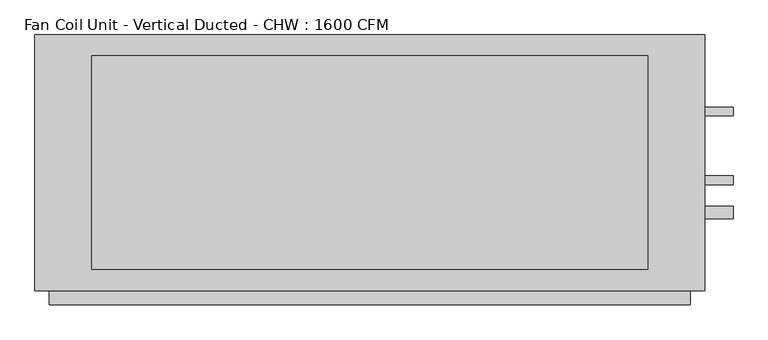
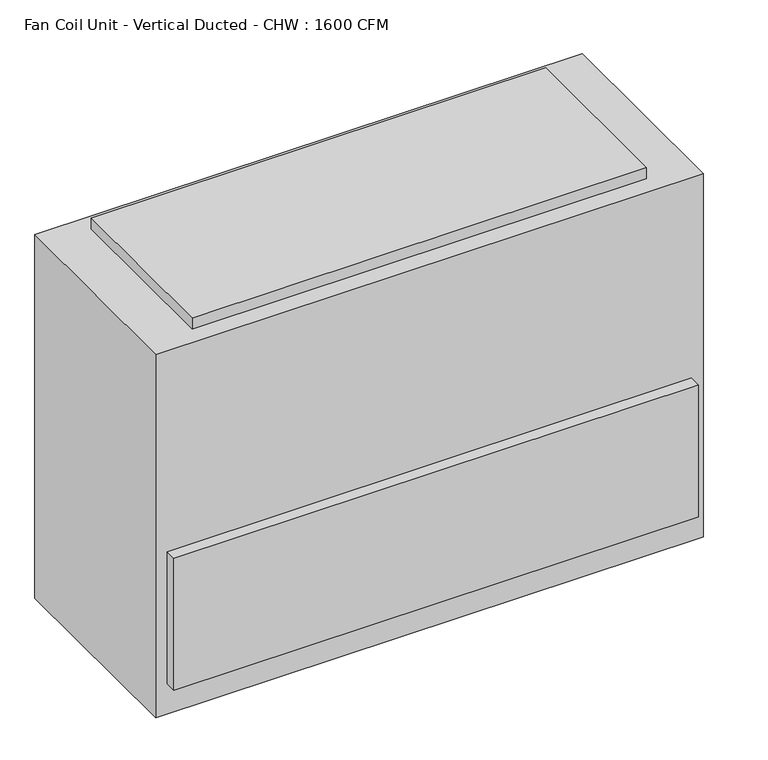
"""IFC4 building model written with IfcOpenShell, lengths in millimetres: proxy geometry, Fan Coil Unit - Vertical Ducted - CHW : 1600 CFM."""

from ifc_helpers import new_model, si_unit, frame, origin, place, context, project, spatial, circle_curve, source, transform, mapped, element, save
from ifc_brep_helpers import plane_surface, cylinder_surface, advanced_brep


def fan_coil_unit_vertical_ducted_chw_1600_cfm_fc1786a7(model_context):
    return source(origin(), model_context, "Body", "AdvancedBrep", [
        advanced_brep(
        [(1092.2, 419.1, 863.6), (101.6, 419.1, 863.6), (101.6, 38.1, 863.6), (1092.2, 38.1, 863.6), (1092.2, 419.1, 838.2), (101.6, 419.1, 838.2), (101.6, 38.1, 838.2), (1092.2, 38.1, 838.2), (1193.8, 455.901774, 838.2), (0.0, 455.901774, 838.2), (0.0, 0.0, 838.2), (1193.8, 0.0, 838.2), (1193.8, 455.901774, 0.0), (1193.8, 0.0, 0.0), (0.0, 0.0, 0.0), (0.0, 455.901774, 0.0), (25.4, 0.0, 374.65), (1168.4, 0.0, 374.65), (1168.4, 0.0, 69.85), (25.4, 0.0, 69.85), (1193.8, 327.314274, 673.1), (1193.8, 311.439274, 673.1), (1193.8, 205.076774, 593.725), (1193.8, 189.201774, 593.725), (1193.8, 150.8125, 431.8), (1193.8, 128.5875, 431.8), (1168.4, -25.4, 374.65), (25.4, -25.4, 374.65), (25.4, -25.4, 69.85), (1168.4, -25.4, 69.85), (1244.6, 311.439274, 673.1), (1244.6, 327.314274, 673.1), (1244.6, 189.201774, 593.725), (1244.6, 205.076774, 593.725), (1244.6, 128.5875, 431.8), (1244.6, 150.8125, 431.8)],
        [
            (0, 1),
            (1, 2),
            (2, 3),
            (3, 0),
            (0, 4),
            (4, 5),
            (5, 1),
            (5, 6),
            (6, 2),
            (6, 7),
            (7, 3),
            (7, 4),
            (8, 9),
            (9, 10),
            (10, 11),
            (11, 8),
            (12, 13),
            (13, 14),
            (14, 15),
            (15, 12),
            (8, 12),
            (15, 9),
            (14, 10),
            (13, 11),
            (16, 17),
            (17, 18),
            (18, 19),
            (19, 16),
            (20, 21, circle_curve(frame((1193.8, 319.376774, 673.1), z_axis=(-1.0, 0.0, 0.0), x_axis=(0.0, 1.0, 0.0)), 7.9375)),
            (21, 20, circle_curve(frame((1193.8, 319.376774, 673.1), z_axis=(-1.0, 0.0, 0.0), x_axis=(0.0, 1.0, 0.0)), 7.9375)),
            (22, 23, circle_curve(frame((1193.8, 197.139274, 593.725), z_axis=(-1.0, 0.0, 0.0), x_axis=(0.0, 1.0, 0.0)), 7.9375)),
            (23, 22, circle_curve(frame((1193.8, 197.139274, 593.725), z_axis=(-1.0, 0.0, 0.0), x_axis=(0.0, 1.0, 0.0)), 7.9375)),
            (24, 25, circle_curve(frame((1193.8, 139.7, 431.8), z_axis=(-1.0, 0.0, 0.0), x_axis=(0.0, 1.0, 0.0)), 11.1125)),
            (25, 24, circle_curve(frame((1193.8, 139.7, 431.8), z_axis=(-1.0, 0.0, 0.0), x_axis=(0.0, 1.0, 0.0)), 11.1125)),
            (26, 27),
            (27, 28),
            (28, 29),
            (29, 26),
            (26, 17),
            (16, 27),
            (19, 28),
            (18, 29),
            (30, 31, circle_curve(frame((1244.6, 319.376774, 673.1), z_axis=(1.0, 0.0, 0.0), x_axis=(0.0, 1.0, 0.0)), 7.9375)),
            (31, 30, circle_curve(frame((1244.6, 319.376774, 673.1), z_axis=(1.0, 0.0, 0.0), x_axis=(0.0, 1.0, 0.0)), 7.9375)),
            (30, 21),
            (20, 31),
            (32, 33, circle_curve(frame((1244.6, 197.139274, 593.725), z_axis=(1.0, 0.0, 0.0), x_axis=(0.0, 1.0, 0.0)), 7.9375)),
            (33, 32, circle_curve(frame((1244.6, 197.139274, 593.725), z_axis=(1.0, 0.0, 0.0), x_axis=(0.0, 1.0, 0.0)), 7.9375)),
            (32, 23),
            (22, 33),
            (34, 35, circle_curve(frame((1244.6, 139.7, 431.8), z_axis=(1.0, 0.0, 0.0), x_axis=(0.0, 1.0, 0.0)), 11.1125)),
            (35, 34, circle_curve(frame((1244.6, 139.7, 431.8), z_axis=(1.0, 0.0, 0.0), x_axis=(0.0, 1.0, 0.0)), 11.1125)),
            (34, 25),
            (24, 35),
        ],
        [
            plane_surface(frame((101.6, 419.1, 863.6), z_axis=(0.0, 0.0, 1.0), x_axis=(-1.0, 0.0, 0.0))),
            plane_surface(frame((1092.2, 419.1, 863.6), z_axis=(0.0, 1.0, 0.0), x_axis=(0.0, 0.0, -1.0))),
            plane_surface(frame((101.6, 419.1, 863.6), z_axis=(-1.0, 0.0, 0.0), x_axis=(0.0, 0.0, -1.0))),
            plane_surface(frame((101.6, 38.1, 863.6), z_axis=(0.0, -1.0, 0.0), x_axis=(0.0, 0.0, -1.0))),
            plane_surface(frame((1092.2, 38.1, 863.6), z_axis=(1.0, 0.0, 0.0), x_axis=(0.0, 0.0, -1.0))),
            plane_surface(frame((0.0, 455.901774, 838.2), z_axis=(0.0, 0.0, 1.0), x_axis=(-1.0, 0.0, 0.0))),
            plane_surface(frame((0.0, 455.901774, 0.0), z_axis=(0.0, 0.0, -1.0), x_axis=(1.0, 0.0, 0.0))),
            plane_surface(frame((1193.8, 455.901774, 838.2), z_axis=(0.0, 1.0, 0.0), x_axis=(0.0, 0.0, -1.0))),
            plane_surface(frame((0.0, 455.901774, 838.2), z_axis=(-1.0, 0.0, 0.0), x_axis=(0.0, 0.0, -1.0))),
            plane_surface(frame((0.0, 0.0, 838.2), z_axis=(0.0, -1.0, 0.0), x_axis=(0.0, 0.0, -1.0))),
            plane_surface(frame((1193.8, 0.0, 838.2), z_axis=(1.0, 0.0, 0.0), x_axis=(0.0, 0.0, -1.0))),
            plane_surface(frame((25.4, -25.4, 374.65), z_axis=(0.0, -1.0, 0.0), x_axis=(-1.0, 0.0, 0.0))),
            plane_surface(frame((1168.4, -25.4, 374.65), z_axis=(0.0, 0.0, 1.0), x_axis=(0.0, 1.0, 0.0))),
            plane_surface(frame((25.4, -25.4, 374.65), z_axis=(-1.0, 0.0, 0.0), x_axis=(0.0, 1.0, 0.0))),
            plane_surface(frame((25.4, -25.4, 69.85), z_axis=(0.0, 0.0, -1.0), x_axis=(0.0, 1.0, 0.0))),
            plane_surface(frame((1168.4, -25.4, 69.85), z_axis=(1.0, 0.0, 0.0), x_axis=(0.0, 1.0, 0.0))),
            plane_surface(frame((1244.6, 327.314274, 673.1), z_axis=(1.0, 0.0, 0.0), x_axis=(0.0, 0.0, 1.0))),
            cylinder_surface(frame((1193.8, 319.376774, 673.1), z_axis=(1.0, 0.0, 0.0), x_axis=(0.0, 1.0, 0.0)), 7.9375),
            plane_surface(frame((1244.6, 205.076774, 593.725), z_axis=(1.0, 0.0, 0.0), x_axis=(0.0, 0.0, 1.0))),
            cylinder_surface(frame((1193.8, 197.139274, 593.725), z_axis=(1.0, 0.0, 0.0), x_axis=(0.0, 1.0, 0.0)), 7.9375),
            plane_surface(frame((1244.6, 150.8125, 431.8), z_axis=(1.0, 0.0, 0.0), x_axis=(0.0, 0.0, 1.0))),
            cylinder_surface(frame((1193.8, 139.7, 431.8), z_axis=(1.0, 0.0, 0.0), x_axis=(0.0, 1.0, 0.0)), 11.1125),
        ],
        [
            (0, [[1, 2, 3, 4]]),
            (1, [[-1, 5, 6, 7]]),
            (2, [[-2, -7, 8, 9]]),
            (3, [[-3, -9, 10, 11]]),
            (4, [[-4, -11, 12, -5]]),
            (5, [[13, 14, 15, 16], [-6, -12, -10, -8]]),
            (6, [[17, 18, 19, 20]]),
            (7, [[-13, 21, -20, 22]]),
            (8, [[-14, -22, -19, 23]]),
            (9, [[-15, -23, -18, 24], [25, 26, 27, 28]]),
            (10, [[-16, -24, -17, -21], [29, 30], [31, 32], [33, 34]]),
            (11, [[35, 36, 37, 38]]),
            (12, [[-35, 39, -25, 40]]),
            (13, [[-36, -40, -28, 41]]),
            (14, [[-37, -41, -27, 42]]),
            (15, [[-38, -42, -26, -39]]),
            (16, [[43, 44]]),
            (17, [[-43, 45, -29, 46]]),
            (17, [[-44, -46, -30, -45]]),
            (18, [[47, 48]]),
            (19, [[-47, 49, -31, 50]]),
            (19, [[-48, -50, -32, -49]]),
            (20, [[51, 52]]),
            (21, [[-51, 53, -33, 54]]),
            (21, [[-52, -54, -34, -53]]),
        ],
    ),
    ])


if __name__ == "__main__":
    model = new_model("IFC4")
    model_context = context("Model", 3, world=origin())
    ifc_project = project(units=[si_unit("LENGTHUNIT", "METRE", prefix="MILLI")], contexts=[model_context])
    site = spatial("IfcSite", under=ifc_project)
    building = spatial("IfcBuilding", under=site)
    placement = place(None, origin())
    fan_coil_unit_vertical_ducted_chw_1600_cfm_shape = fan_coil_unit_vertical_ducted_chw_1600_cfm_fc1786a7(model_context)
    element("IfcBuildingElementProxy", 1, Name="Fan Coil Unit - Vertical Ducted - CHW : 1600 CFM", ObjectType="Fan Coil Unit - Vertical Ducted - CHW : 1600 CFM", at=placement, inside=building, context=model_context, shape_type="MappedRepresentation", body=[
        mapped(fan_coil_unit_vertical_ducted_chw_1600_cfm_shape, transform((0.0, 0.0, 0.0), x_axis=(1.0, 0.0, 0.0), y_axis=(0.0, 1.0, 0.0), z_axis=(0.0, 0.0, 1.0))),
    ])
    save(model, "model.ifc")

# Revit data of these elements
# Type "Fan Coil Unit - Vertical Ducted - CHW : 1600 CFM"
#   COBie.Type.CreatedBy = "design@eagle.com"
#   COBie.Type.CreatedOn = "2016-10-27T05:31:12"
#   COBie.Type.Name = "Fan Coil Unit - Vertical Ducted - CHW_1600 CFM"
#   COBie.Type.Category = "23-75 70 17 27 : Fan Coil Units"
#   COBie.Type.Description = "Fan Coil Unit - Vertical Ducted - CHW_1600 CFM"
#   COBie.Type.Manufacturer = ""
#   COBie.Type.ModelNumber = ""
#   COBie.Type.ReplacementCost = 0
#   Water Pressure Drop [instance default] = 25.00 psi
#   Voltage = 240 V
#   Unit Length = 3' - 11"
#   Total Cooling Capacity = 64700 Btu/h
#   Supply Air Width = 39"
#   Sensible Cooling Capacity = 43600 Btu/h
#   Return Air Width = 45"
#   Nominal Air Flow [instance default] = 1600 CFM
#   External Static Pressure [instance default] = 0.30 in-wg
#   Drain Flow [instance default] = 0 GPM
#   Chilled Water Flow [instance default] = 15 GPM
#   C2 Offset 1 = 0' - 5 3/8"
#   Apparent Load = 900 VA
#   COBie.Type = yes
#   Number of Poles = 2
#   Load Classification = Cooling
#   CFU Material = none
